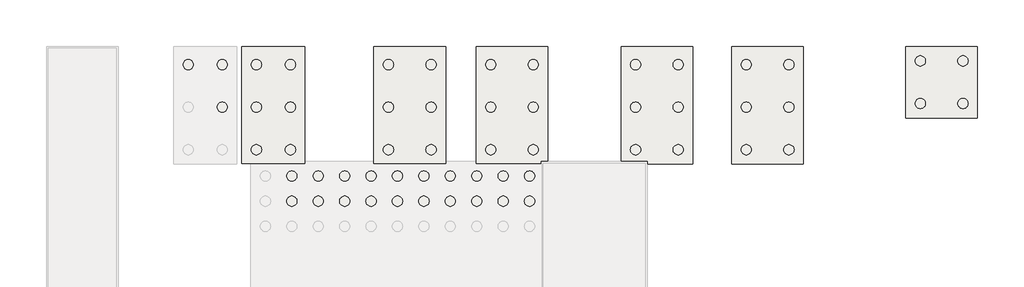
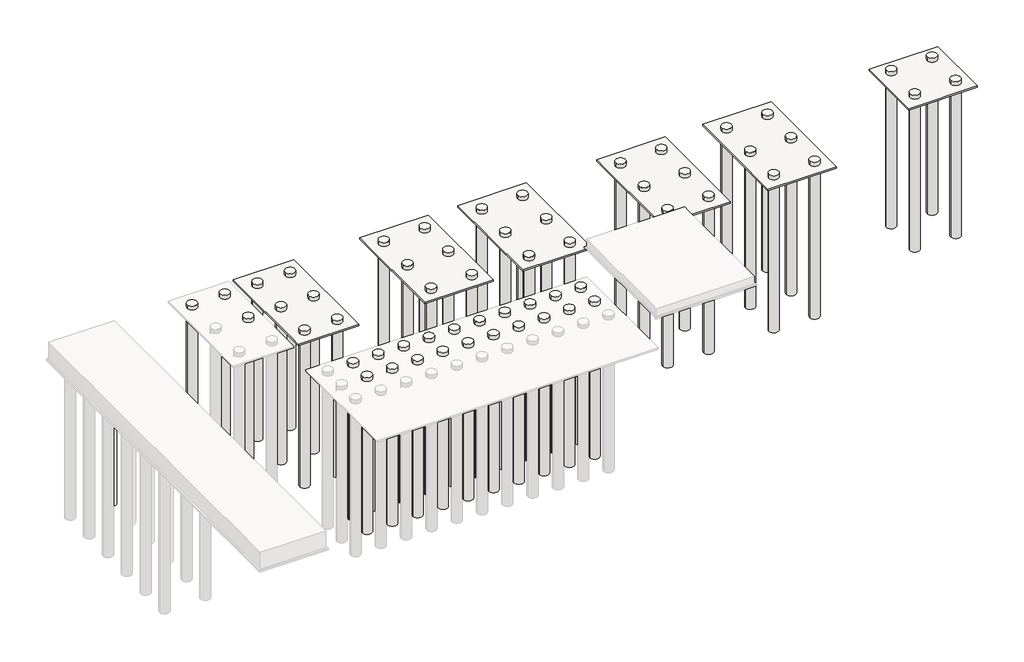
# One storey, part 3 of 3: 64 slabs.
"""IFC4 building model written with IfcOpenShell, lengths in millimetres."""

from ifc_helpers import new_model, si_unit, point, frame, frame_2d, origin, place, context, project, spatial, polyline, circle_curve, trimmed, segment, composite_curve, outline, extrude, faceted_brep, element, save

model = new_model("IFC4")

# Units and contexts
model_context = context("Model", 3, world=origin())
ifc_project = project(units=[si_unit("LENGTHUNIT", "METRE", prefix="MILLI")], contexts=[model_context])

# Site, building, storey
site = spatial("IfcSite", under=ifc_project)
building = spatial("IfcBuilding", under=site)
storey = spatial("IfcBuildingStorey", under=building, Name="B.O.F(FDN)", Elevation=-2500.0279945)

# Slabs
placement = place(None, origin())
element("IfcSlab", 1, ObjectType="H_SF_ACF_Lean_T100", at=placement, inside=storey, context=model_context, shape_type="SweptSolid", body=[
    extrude(outline(polyline([(37900.0, 41319.5208589), (42100.0, 41319.5208589), (42100.0, 34399.5208589), (37900.0, 34399.5208589), (37900.0, 41319.5208589)])), frame((0.0, 0.0, -2600.0279945), z_axis=(0.0, 0.0, 1.0), x_axis=(1.0, 0.0, 0.0)), (0.0, 0.0, 1.0), 100.0),
])
element("IfcSlab", 2, ObjectType="H_SF_ACF_Lean_T100", at=placement, inside=storey, context=model_context, shape_type="SweptSolid", body=[
    extrude(outline(polyline([(48115.0, 41319.5208589), (52315.0, 41319.5208589), (52315.0, 37119.5208589), (48115.0, 37119.5208589), (48115.0, 41319.5208589)])), frame((0.0, 0.0, -2600.0279945), z_axis=(0.0, 0.0, 1.0), x_axis=(1.0, 0.0, 0.0)), (0.0, 0.0, 1.0), 100.0),
])
element("IfcSlab", 3, ObjectType="H_SF_ACF_Lean_T100", at=placement, inside=storey, context=model_context, shape_type="SweptSolid", body=[
    extrude(outline(polyline([(31400.0, 41319.5208589), (35600.0, 41319.5208589), (35600.0, 34399.5208589), (31400.0, 34399.5208589), (31400.0, 41319.5208589)])), frame((0.0, 0.0, -2600.0279945), z_axis=(0.0, 0.0, 1.0), x_axis=(1.0, 0.0, 0.0)), (0.0, 0.0, 1.0), 100.0),
])
element("IfcSlab", 4, ObjectType="H_SF_ACF_Lean_T100", at=placement, inside=storey, context=model_context, shape_type="SweptSolid", body=[
    extrude(outline(polyline([(9150.0, 41319.5208589), (12850.0, 41319.5208589), (12850.0, 34449.5208589), (9150.0, 34449.5208589), (9150.0, 41319.5208589)])), frame((0.0, 0.0, -2600.0279945), z_axis=(0.0, 0.0, 1.0), x_axis=(1.0, 0.0, 0.0)), (0.0, 0.0, 1.0), 100.0),
])
element("IfcSlab", 5, ObjectType="H_SF_ACF_Lean_T100", at=placement, inside=storey, context=model_context, shape_type="SweptSolid", body=[
    extrude(outline(polyline([(21100.0, 41319.5208589), (21100.0, 34449.5208589), (16900.0, 34449.5208589), (16900.0, 41319.5208589), (21100.0, 41319.5208589)])), frame((0.0, 0.0, -2600.0279945), z_axis=(0.0, 0.0, 1.0), x_axis=(1.0, 0.0, 0.0)), (0.0, 0.0, 1.0), 100.0),
])
element("IfcSlab", 6, ObjectType="H_SF_ACF_Lean_T100", at=placement, inside=storey, context=model_context, shape_type="Brep", body=[
    faceted_brep([(27100.0, 41319.5208589, -2600.0279945), (27100.0, 34449.5208589, -2600.0279945), (22900.0, 34449.5208589, -2600.0279945), (22900.0, 41319.5208589, -2600.0279945), (27100.0, 41319.5208589, -2500.0279945), (22900.0, 41319.5208589, -2500.0279945), (22900.0, 34449.5208589, -2500.0279945), (26730.0, 34449.5208589, -2500.0279945), (26780.0, 34449.5208589, -2500.0279945), (27100.0, 34449.5208589, -2500.0279945)], [[[0, 1, 2, 3]], [[4, 5, 6, 7, 8, 9]], [[1, 0, 4, 9]], [[2, 1, 9, 8, 7, 6]], [[3, 2, 6, 5]], [[0, 3, 5, 4]]]),
])
element("IfcSlab", 7, ObjectType="Pile : H_SF_API_Steel Pile D508x12t_L10m", at=placement, inside=storey, context=model_context, shape_type="SweptSolid", body=[
    extrude(outline(composite_curve([segment(trimmed(circle_curve(frame_2d((1035.0, 40249.5208589)), 300.0), [point((1335.0, 40249.5208589))], [point((735.0, 40249.5208589))], False, "CARTESIAN"), True, "CONTINUOUS"), segment(trimmed(circle_curve(frame_2d((1035.0, 40249.5208589)), 300.0), [point((735.0, 40249.5208589))], [point((1335.0, 40249.5208589))], False, "CARTESIAN"), True, "CONTINUOUS")], self_intersect=False)), frame((0.0, 0.0, -13500.0279945), z_axis=(0.0, 0.0, 1.0), x_axis=(1.0, 0.0, 0.0)), (0.0, 0.0, 1.0), 10150.0),
])
element("IfcSlab", 8, ObjectType="Pile : H_SF_API_Steel Pile D508x12t_L10m", at=placement, inside=storey, context=model_context, shape_type="SweptSolid", body=[
    extrude(outline(composite_curve([segment(trimmed(circle_curve(frame_2d((51465.0, 37969.5208589)), 300.0), [point((51765.0, 37969.5208589))], [point((51165.0, 37969.5208589))], False, "CARTESIAN"), True, "CONTINUOUS"), segment(trimmed(circle_curve(frame_2d((51465.0, 37969.5208589)), 300.0), [point((51165.0, 37969.5208589))], [point((51765.0, 37969.5208589))], False, "CARTESIAN"), True, "CONTINUOUS")], self_intersect=False)), frame((0.0, 0.0, -12400.0279945), z_axis=(0.0, 0.0, 1.0), x_axis=(1.0, 0.0, 0.0)), (0.0, 0.0, 1.0), 10150.0),
])
element("IfcSlab", 9, ObjectType="Pile : H_SF_API_Steel Pile D508x12t_L10m", at=placement, inside=storey, context=model_context, shape_type="SweptSolid", body=[
    extrude(outline(composite_curve([segment(trimmed(circle_curve(frame_2d((48965.0, 37969.5208589)), 300.0), [point((48665.0, 37969.5208589))], [point((49265.0, 37969.5208589))], False, "CARTESIAN"), True, "CONTINUOUS"), segment(trimmed(circle_curve(frame_2d((48965.0, 37969.5208589)), 300.0), [point((49265.0, 37969.5208589))], [point((48665.0, 37969.5208589))], False, "CARTESIAN"), True, "CONTINUOUS")], self_intersect=False)), frame((0.0, 0.0, -12400.0279945), z_axis=(0.0, 0.0, 1.0), x_axis=(1.0, 0.0, 0.0)), (0.0, 0.0, 1.0), 10150.0),
])
element("IfcSlab", 10, ObjectType="Pile : H_SF_API_Steel Pile D508x12t_L10m", at=placement, inside=storey, context=model_context, shape_type="SweptSolid", body=[
    extrude(outline(composite_curve([segment(trimmed(circle_curve(frame_2d((51465.0, 40469.5208589)), 300.0), [point((51765.0, 40469.5208589))], [point((51165.0, 40469.5208589))], False, "CARTESIAN"), True, "CONTINUOUS"), segment(trimmed(circle_curve(frame_2d((51465.0, 40469.5208589)), 300.0), [point((51165.0, 40469.5208589))], [point((51765.0, 40469.5208589))], False, "CARTESIAN"), True, "CONTINUOUS")], self_intersect=False)), frame((0.0, 0.0, -12400.0279945), z_axis=(0.0, 0.0, 1.0), x_axis=(1.0, 0.0, 0.0)), (0.0, 0.0, 1.0), 10150.0),
])
element("IfcSlab", 11, ObjectType="Pile : H_SF_API_Steel Pile D508x12t_L10m", at=placement, inside=storey, context=model_context, shape_type="SweptSolid", body=[
    extrude(outline(composite_curve([segment(trimmed(circle_curve(frame_2d((48965.0, 40469.5208589)), 300.0), [point((48665.0, 40469.5208589))], [point((49265.0, 40469.5208589))], False, "CARTESIAN"), True, "CONTINUOUS"), segment(trimmed(circle_curve(frame_2d((48965.0, 40469.5208589)), 300.0), [point((49265.0, 40469.5208589))], [point((48665.0, 40469.5208589))], False, "CARTESIAN"), True, "CONTINUOUS")], self_intersect=False)), frame((0.0, 0.0, -12400.0279945), z_axis=(0.0, 0.0, 1.0), x_axis=(1.0, 0.0, 0.0)), (0.0, 0.0, 1.0), 10150.0),
])
element("IfcSlab", 12, ObjectType="Pile : H_SF_API_Steel Pile D508x12t_L10m", at=placement, inside=storey, context=model_context, shape_type="SweptSolid", body=[
    extrude(outline(composite_curve([segment(trimmed(circle_curve(frame_2d((6000.0, 40249.5208589)), 300.0), [point((5700.0, 40249.5208589))], [point((6300.0, 40249.5208589))], False, "CARTESIAN"), True, "CONTINUOUS"), segment(trimmed(circle_curve(frame_2d((6000.0, 40249.5208589)), 300.0), [point((6300.0, 40249.5208589))], [point((5700.0, 40249.5208589))], False, "CARTESIAN"), True, "CONTINUOUS")], self_intersect=False)), frame((0.0, 0.0, -12400.0279945), z_axis=(0.0, 0.0, 1.0), x_axis=(1.0, 0.0, 0.0)), (0.0, 0.0, 1.0), 10150.0),
])
element("IfcSlab", 13, ObjectType="Pile : H_SF_API_Steel Pile D508x12t_L10m", at=placement, inside=storey, context=model_context, shape_type="SweptSolid", body=[
    extrude(outline(composite_curve([segment(trimmed(circle_curve(frame_2d((8000.0, 40249.5208589)), 300.0), [point((8300.0, 40249.5208589))], [point((7700.0, 40249.5208589))], False, "CARTESIAN"), True, "CONTINUOUS"), segment(trimmed(circle_curve(frame_2d((8000.0, 40249.5208589)), 300.0), [point((7700.0, 40249.5208589))], [point((8300.0, 40249.5208589))], False, "CARTESIAN"), True, "CONTINUOUS")], self_intersect=False)), frame((0.0, 0.0, -12400.0279945), z_axis=(0.0, 0.0, 1.0), x_axis=(1.0, 0.0, 0.0)), (0.0, 0.0, 1.0), 10150.0),
])
element("IfcSlab", 14, ObjectType="Pile : H_SF_API_Steel Pile D508x12t_L10m", at=placement, inside=storey, context=model_context, shape_type="SweptSolid", body=[
    extrude(outline(composite_curve([segment(trimmed(circle_curve(frame_2d((8000.0, 37749.5208589)), 300.0), [point((8300.0, 37749.5208589))], [point((7700.0, 37749.5208589))], False, "CARTESIAN"), True, "CONTINUOUS"), segment(trimmed(circle_curve(frame_2d((8000.0, 37749.5208589)), 300.0), [point((7700.0, 37749.5208589))], [point((8300.0, 37749.5208589))], False, "CARTESIAN"), True, "CONTINUOUS")], self_intersect=False)), frame((0.0, 0.0, -12400.0279945), z_axis=(0.0, 0.0, 1.0), x_axis=(1.0, 0.0, 0.0)), (0.0, 0.0, 1.0), 10150.0),
])
element("IfcSlab", 15, ObjectType="Pile : H_SF_API_Steel Pile D508x12t_L10m", at=placement, inside=storey, context=model_context, shape_type="SweptSolid", body=[
    extrude(outline(composite_curve([segment(trimmed(circle_curve(frame_2d((10000.0, 40249.5208589)), 300.0), [point((9700.0, 40249.5208589))], [point((10300.0, 40249.5208589))], False, "CARTESIAN"), True, "CONTINUOUS"), segment(trimmed(circle_curve(frame_2d((10000.0, 40249.5208589)), 300.0), [point((10300.0, 40249.5208589))], [point((9700.0, 40249.5208589))], False, "CARTESIAN"), True, "CONTINUOUS")], self_intersect=False)), frame((0.0, 0.0, -12400.0279945), z_axis=(0.0, 0.0, 1.0), x_axis=(1.0, 0.0, 0.0)), (0.0, 0.0, 1.0), 10150.0),
])
element("IfcSlab", 16, ObjectType="Pile : H_SF_API_Steel Pile D508x12t_L10m", at=placement, inside=storey, context=model_context, shape_type="SweptSolid", body=[
    extrude(outline(composite_curve([segment(trimmed(circle_curve(frame_2d((12000.0, 40249.5208589)), 300.0), [point((12300.0, 40249.5208589))], [point((11700.0, 40249.5208589))], False, "CARTESIAN"), True, "CONTINUOUS"), segment(trimmed(circle_curve(frame_2d((12000.0, 40249.5208589)), 300.0), [point((11700.0, 40249.5208589))], [point((12300.0, 40249.5208589))], False, "CARTESIAN"), True, "CONTINUOUS")], self_intersect=False)), frame((0.0, 0.0, -12400.0279945), z_axis=(0.0, 0.0, 1.0), x_axis=(1.0, 0.0, 0.0)), (0.0, 0.0, 1.0), 10150.0),
])
element("IfcSlab", 17, ObjectType="Pile : H_SF_API_Steel Pile D508x12t_L10m", at=placement, inside=storey, context=model_context, shape_type="SweptSolid", body=[
    extrude(outline(composite_curve([segment(trimmed(circle_curve(frame_2d((10000.0, 37749.5208589)), 300.0), [point((9700.0, 37749.5208589))], [point((10300.0, 37749.5208589))], False, "CARTESIAN"), True, "CONTINUOUS"), segment(trimmed(circle_curve(frame_2d((10000.0, 37749.5208589)), 300.0), [point((10300.0, 37749.5208589))], [point((9700.0, 37749.5208589))], False, "CARTESIAN"), True, "CONTINUOUS")], self_intersect=False)), frame((0.0, 0.0, -12400.0279945), z_axis=(0.0, 0.0, 1.0), x_axis=(1.0, 0.0, 0.0)), (0.0, 0.0, 1.0), 10150.0),
])
element("IfcSlab", 18, ObjectType="Pile : H_SF_API_Steel Pile D508x12t_L10m", at=placement, inside=storey, context=model_context, shape_type="SweptSolid", body=[
    extrude(outline(composite_curve([segment(trimmed(circle_curve(frame_2d((12000.0, 37749.5208589)), 300.0), [point((12300.0, 37749.5208589))], [point((11700.0, 37749.5208589))], False, "CARTESIAN"), True, "CONTINUOUS"), segment(trimmed(circle_curve(frame_2d((12000.0, 37749.5208589)), 300.0), [point((11700.0, 37749.5208589))], [point((12300.0, 37749.5208589))], False, "CARTESIAN"), True, "CONTINUOUS")], self_intersect=False)), frame((0.0, 0.0, -12400.0279945), z_axis=(0.0, 0.0, 1.0), x_axis=(1.0, 0.0, 0.0)), (0.0, 0.0, 1.0), 10150.0),
])
element("IfcSlab", 19, ObjectType="Pile : H_SF_API_Steel Pile D508x12t_L10m", at=placement, inside=storey, context=model_context, shape_type="SweptSolid", body=[
    extrude(outline(composite_curve([segment(trimmed(circle_curve(frame_2d((10000.0, 35249.5208589)), 300.0), [point((9700.0, 35249.5208589))], [point((10300.0, 35249.5208589))], False, "CARTESIAN"), True, "CONTINUOUS"), segment(trimmed(circle_curve(frame_2d((10000.0, 35249.5208589)), 300.0), [point((10300.0, 35249.5208589))], [point((9700.0, 35249.5208589))], False, "CARTESIAN"), True, "CONTINUOUS")], self_intersect=False)), frame((0.0, 0.0, -12400.0279945), z_axis=(0.0, 0.0, 1.0), x_axis=(1.0, 0.0, 0.0)), (0.0, 0.0, 1.0), 10150.0),
])
element("IfcSlab", 20, ObjectType="Pile : H_SF_API_Steel Pile D508x12t_L10m", at=placement, inside=storey, context=model_context, shape_type="SweptSolid", body=[
    extrude(outline(composite_curve([segment(trimmed(circle_curve(frame_2d((12000.0, 35249.5208589)), 300.0), [point((12300.0, 35249.5208589))], [point((11700.0, 35249.5208589))], False, "CARTESIAN"), True, "CONTINUOUS"), segment(trimmed(circle_curve(frame_2d((12000.0, 35249.5208589)), 300.0), [point((11700.0, 35249.5208589))], [point((12300.0, 35249.5208589))], False, "CARTESIAN"), True, "CONTINUOUS")], self_intersect=False)), frame((0.0, 0.0, -12400.0279945), z_axis=(0.0, 0.0, 1.0), x_axis=(1.0, 0.0, 0.0)), (0.0, 0.0, 1.0), 10150.0),
])
element("IfcSlab", 21, ObjectType="Pile : H_SF_API_Steel Pile D508x12t_L10m", at=placement, inside=storey, context=model_context, shape_type="SweptSolid", body=[
    extrude(outline(composite_curve([segment(trimmed(circle_curve(frame_2d((20250.0, 40249.5208589)), 300.0), [point((20550.0, 40249.5208589))], [point((19950.0, 40249.5208589))], False, "CARTESIAN"), True, "CONTINUOUS"), segment(trimmed(circle_curve(frame_2d((20250.0, 40249.5208589)), 300.0), [point((19950.0, 40249.5208589))], [point((20550.0, 40249.5208589))], False, "CARTESIAN"), True, "CONTINUOUS")], self_intersect=False)), frame((0.0, 0.0, -12400.0279945), z_axis=(0.0, 0.0, 1.0), x_axis=(1.0, 0.0, 0.0)), (0.0, 0.0, 1.0), 10150.0),
])
element("IfcSlab", 22, ObjectType="Pile : H_SF_API_Steel Pile D508x12t_L10m", at=placement, inside=storey, context=model_context, shape_type="SweptSolid", body=[
    extrude(outline(composite_curve([segment(trimmed(circle_curve(frame_2d((17750.0, 40249.5208589)), 300.0), [point((17450.0, 40249.5208589))], [point((18050.0, 40249.5208589))], False, "CARTESIAN"), True, "CONTINUOUS"), segment(trimmed(circle_curve(frame_2d((17750.0, 40249.5208589)), 300.0), [point((18050.0, 40249.5208589))], [point((17450.0, 40249.5208589))], False, "CARTESIAN"), True, "CONTINUOUS")], self_intersect=False)), frame((0.0, 0.0, -12400.0279945), z_axis=(0.0, 0.0, 1.0), x_axis=(1.0, 0.0, 0.0)), (0.0, 0.0, 1.0), 10150.0),
])
element("IfcSlab", 23, ObjectType="Pile : H_SF_API_Steel Pile D508x12t_L10m", at=placement, inside=storey, context=model_context, shape_type="SweptSolid", body=[
    extrude(outline(composite_curve([segment(trimmed(circle_curve(frame_2d((20250.0, 37749.5208589)), 300.0), [point((20550.0, 37749.5208589))], [point((19950.0, 37749.5208589))], False, "CARTESIAN"), True, "CONTINUOUS"), segment(trimmed(circle_curve(frame_2d((20250.0, 37749.5208589)), 300.0), [point((19950.0, 37749.5208589))], [point((20550.0, 37749.5208589))], False, "CARTESIAN"), True, "CONTINUOUS")], self_intersect=False)), frame((0.0, 0.0, -12400.0279945), z_axis=(0.0, 0.0, 1.0), x_axis=(1.0, 0.0, 0.0)), (0.0, 0.0, 1.0), 10150.0),
])
element("IfcSlab", 24, ObjectType="Pile : H_SF_API_Steel Pile D508x12t_L10m", at=placement, inside=storey, context=model_context, shape_type="SweptSolid", body=[
    extrude(outline(composite_curve([segment(trimmed(circle_curve(frame_2d((17750.0, 37749.5208589)), 300.0), [point((17450.0, 37749.5208589))], [point((18050.0, 37749.5208589))], False, "CARTESIAN"), True, "CONTINUOUS"), segment(trimmed(circle_curve(frame_2d((17750.0, 37749.5208589)), 300.0), [point((18050.0, 37749.5208589))], [point((17450.0, 37749.5208589))], False, "CARTESIAN"), True, "CONTINUOUS")], self_intersect=False)), frame((0.0, 0.0, -12400.0279945), z_axis=(0.0, 0.0, 1.0), x_axis=(1.0, 0.0, 0.0)), (0.0, 0.0, 1.0), 10150.0),
])
element("IfcSlab", 25, ObjectType="Pile : H_SF_API_Steel Pile D508x12t_L10m", at=placement, inside=storey, context=model_context, shape_type="SweptSolid", body=[
    extrude(outline(composite_curve([segment(trimmed(circle_curve(frame_2d((20250.0, 35249.5208589)), 300.0), [point((20550.0, 35249.5208589))], [point((19950.0, 35249.5208589))], False, "CARTESIAN"), True, "CONTINUOUS"), segment(trimmed(circle_curve(frame_2d((20250.0, 35249.5208589)), 300.0), [point((19950.0, 35249.5208589))], [point((20550.0, 35249.5208589))], False, "CARTESIAN"), True, "CONTINUOUS")], self_intersect=False)), frame((0.0, 0.0, -12400.0279945), z_axis=(0.0, 0.0, 1.0), x_axis=(1.0, 0.0, 0.0)), (0.0, 0.0, 1.0), 10150.0),
])
element("IfcSlab", 26, ObjectType="Pile : H_SF_API_Steel Pile D508x12t_L10m", at=placement, inside=storey, context=model_context, shape_type="SweptSolid", body=[
    extrude(outline(composite_curve([segment(trimmed(circle_curve(frame_2d((17750.0, 35249.5208589)), 300.0), [point((17450.0, 35249.5208589))], [point((18050.0, 35249.5208589))], False, "CARTESIAN"), True, "CONTINUOUS"), segment(trimmed(circle_curve(frame_2d((17750.0, 35249.5208589)), 300.0), [point((18050.0, 35249.5208589))], [point((17450.0, 35249.5208589))], False, "CARTESIAN"), True, "CONTINUOUS")], self_intersect=False)), frame((0.0, 0.0, -12400.0279945), z_axis=(0.0, 0.0, 1.0), x_axis=(1.0, 0.0, 0.0)), (0.0, 0.0, 1.0), 10150.0),
])
element("IfcSlab", 27, ObjectType="Pile : H_SF_API_Steel Pile D508x12t_L10m", at=placement, inside=storey, context=model_context, shape_type="SweptSolid", body=[
    extrude(outline(composite_curve([segment(trimmed(circle_curve(frame_2d((26250.0, 40249.5208589)), 300.0), [point((26550.0, 40249.5208589))], [point((25950.0, 40249.5208589))], False, "CARTESIAN"), True, "CONTINUOUS"), segment(trimmed(circle_curve(frame_2d((26250.0, 40249.5208589)), 300.0), [point((25950.0, 40249.5208589))], [point((26550.0, 40249.5208589))], False, "CARTESIAN"), True, "CONTINUOUS")], self_intersect=False)), frame((0.0, 0.0, -12400.0279945), z_axis=(0.0, 0.0, 1.0), x_axis=(1.0, 0.0, 0.0)), (0.0, 0.0, 1.0), 10150.0),
])
element("IfcSlab", 28, ObjectType="Pile : H_SF_API_Steel Pile D508x12t_L10m", at=placement, inside=storey, context=model_context, shape_type="SweptSolid", body=[
    extrude(outline(composite_curve([segment(trimmed(circle_curve(frame_2d((23750.0, 40249.5208589)), 300.0), [point((23450.0, 40249.5208589))], [point((24050.0, 40249.5208589))], False, "CARTESIAN"), True, "CONTINUOUS"), segment(trimmed(circle_curve(frame_2d((23750.0, 40249.5208589)), 300.0), [point((24050.0, 40249.5208589))], [point((23450.0, 40249.5208589))], False, "CARTESIAN"), True, "CONTINUOUS")], self_intersect=False)), frame((0.0, 0.0, -12400.0279945), z_axis=(0.0, 0.0, 1.0), x_axis=(1.0, 0.0, 0.0)), (0.0, 0.0, 1.0), 10150.0),
])
element("IfcSlab", 29, ObjectType="Pile : H_SF_API_Steel Pile D508x12t_L10m", at=placement, inside=storey, context=model_context, shape_type="SweptSolid", body=[
    extrude(outline(composite_curve([segment(trimmed(circle_curve(frame_2d((26250.0, 37749.5208589)), 300.0), [point((26550.0, 37749.5208589))], [point((25950.0, 37749.5208589))], False, "CARTESIAN"), True, "CONTINUOUS"), segment(trimmed(circle_curve(frame_2d((26250.0, 37749.5208589)), 300.0), [point((25950.0, 37749.5208589))], [point((26550.0, 37749.5208589))], False, "CARTESIAN"), True, "CONTINUOUS")], self_intersect=False)), frame((0.0, 0.0, -12400.0279945), z_axis=(0.0, 0.0, 1.0), x_axis=(1.0, 0.0, 0.0)), (0.0, 0.0, 1.0), 10150.0),
])
element("IfcSlab", 30, ObjectType="Pile : H_SF_API_Steel Pile D508x12t_L10m", at=placement, inside=storey, context=model_context, shape_type="SweptSolid", body=[
    extrude(outline(composite_curve([segment(trimmed(circle_curve(frame_2d((23750.0, 37749.5208589)), 300.0), [point((23450.0, 37749.5208589))], [point((24050.0, 37749.5208589))], False, "CARTESIAN"), True, "CONTINUOUS"), segment(trimmed(circle_curve(frame_2d((23750.0, 37749.5208589)), 300.0), [point((24050.0, 37749.5208589))], [point((23450.0, 37749.5208589))], False, "CARTESIAN"), True, "CONTINUOUS")], self_intersect=False)), frame((0.0, 0.0, -12400.0279945), z_axis=(0.0, 0.0, 1.0), x_axis=(1.0, 0.0, 0.0)), (0.0, 0.0, 1.0), 10150.0),
])
element("IfcSlab", 31, ObjectType="Pile : H_SF_API_Steel Pile D508x12t_L10m", at=placement, inside=storey, context=model_context, shape_type="SweptSolid", body=[
    extrude(outline(composite_curve([segment(trimmed(circle_curve(frame_2d((26250.0, 35249.5208589)), 300.0), [point((26550.0, 35249.5208589))], [point((25950.0, 35249.5208589))], False, "CARTESIAN"), True, "CONTINUOUS"), segment(trimmed(circle_curve(frame_2d((26250.0, 35249.5208589)), 300.0), [point((25950.0, 35249.5208589))], [point((26550.0, 35249.5208589))], False, "CARTESIAN"), True, "CONTINUOUS")], self_intersect=False)), frame((0.0, 0.0, -12400.0279945), z_axis=(0.0, 0.0, 1.0), x_axis=(1.0, 0.0, 0.0)), (0.0, 0.0, 1.0), 10150.0),
])
element("IfcSlab", 32, ObjectType="Pile : H_SF_API_Steel Pile D508x12t_L10m", at=placement, inside=storey, context=model_context, shape_type="SweptSolid", body=[
    extrude(outline(composite_curve([segment(trimmed(circle_curve(frame_2d((23750.0, 35249.5208589)), 300.0), [point((23450.0, 35249.5208589))], [point((24050.0, 35249.5208589))], False, "CARTESIAN"), True, "CONTINUOUS"), segment(trimmed(circle_curve(frame_2d((23750.0, 35249.5208589)), 300.0), [point((24050.0, 35249.5208589))], [point((23450.0, 35249.5208589))], False, "CARTESIAN"), True, "CONTINUOUS")], self_intersect=False)), frame((0.0, 0.0, -12400.0279945), z_axis=(0.0, 0.0, 1.0), x_axis=(1.0, 0.0, 0.0)), (0.0, 0.0, 1.0), 10150.0),
])
element("IfcSlab", 33, ObjectType="Pile : H_SF_API_Steel Pile D508x12t_L10m", at=placement, inside=storey, context=model_context, shape_type="SweptSolid", body=[
    extrude(outline(composite_curve([segment(trimmed(circle_curve(frame_2d((34750.0, 40249.5208589)), 300.0), [point((35050.0, 40249.5208589))], [point((34450.0, 40249.5208589))], False, "CARTESIAN"), True, "CONTINUOUS"), segment(trimmed(circle_curve(frame_2d((34750.0, 40249.5208589)), 300.0), [point((34450.0, 40249.5208589))], [point((35050.0, 40249.5208589))], False, "CARTESIAN"), True, "CONTINUOUS")], self_intersect=False)), frame((0.0, 0.0, -12400.0279945), z_axis=(0.0, 0.0, 1.0), x_axis=(1.0, 0.0, 0.0)), (0.0, 0.0, 1.0), 10150.0),
])
element("IfcSlab", 34, ObjectType="Pile : H_SF_API_Steel Pile D508x12t_L10m", at=placement, inside=storey, context=model_context, shape_type="SweptSolid", body=[
    extrude(outline(composite_curve([segment(trimmed(circle_curve(frame_2d((32250.0, 40249.5208589)), 300.0), [point((31950.0, 40249.5208589))], [point((32550.0, 40249.5208589))], False, "CARTESIAN"), True, "CONTINUOUS"), segment(trimmed(circle_curve(frame_2d((32250.0, 40249.5208589)), 300.0), [point((32550.0, 40249.5208589))], [point((31950.0, 40249.5208589))], False, "CARTESIAN"), True, "CONTINUOUS")], self_intersect=False)), frame((0.0, 0.0, -12400.0279945), z_axis=(0.0, 0.0, 1.0), x_axis=(1.0, 0.0, 0.0)), (0.0, 0.0, 1.0), 10150.0),
])
element("IfcSlab", 35, ObjectType="Pile : H_SF_API_Steel Pile D508x12t_L10m", at=placement, inside=storey, context=model_context, shape_type="SweptSolid", body=[
    extrude(outline(composite_curve([segment(trimmed(circle_curve(frame_2d((34750.0, 37749.5208589)), 300.0), [point((35050.0, 37749.5208589))], [point((34450.0, 37749.5208589))], False, "CARTESIAN"), True, "CONTINUOUS"), segment(trimmed(circle_curve(frame_2d((34750.0, 37749.5208589)), 300.0), [point((34450.0, 37749.5208589))], [point((35050.0, 37749.5208589))], False, "CARTESIAN"), True, "CONTINUOUS")], self_intersect=False)), frame((0.0, 0.0, -12400.0279945), z_axis=(0.0, 0.0, 1.0), x_axis=(1.0, 0.0, 0.0)), (0.0, 0.0, 1.0), 10150.0),
])
element("IfcSlab", 36, ObjectType="Pile : H_SF_API_Steel Pile D508x12t_L10m", at=placement, inside=storey, context=model_context, shape_type="SweptSolid", body=[
    extrude(outline(composite_curve([segment(trimmed(circle_curve(frame_2d((32250.0, 37749.5208589)), 300.0), [point((31950.0, 37749.5208589))], [point((32550.0, 37749.5208589))], False, "CARTESIAN"), True, "CONTINUOUS"), segment(trimmed(circle_curve(frame_2d((32250.0, 37749.5208589)), 300.0), [point((32550.0, 37749.5208589))], [point((31950.0, 37749.5208589))], False, "CARTESIAN"), True, "CONTINUOUS")], self_intersect=False)), frame((0.0, 0.0, -12400.0279945), z_axis=(0.0, 0.0, 1.0), x_axis=(1.0, 0.0, 0.0)), (0.0, 0.0, 1.0), 10150.0),
])
element("IfcSlab", 37, ObjectType="Pile : H_SF_API_Steel Pile D508x12t_L10m", at=placement, inside=storey, context=model_context, shape_type="SweptSolid", body=[
    extrude(outline(composite_curve([segment(trimmed(circle_curve(frame_2d((34750.0, 35249.5208589)), 300.0), [point((35050.0, 35249.5208589))], [point((34450.0, 35249.5208589))], False, "CARTESIAN"), True, "CONTINUOUS"), segment(trimmed(circle_curve(frame_2d((34750.0, 35249.5208589)), 300.0), [point((34450.0, 35249.5208589))], [point((35050.0, 35249.5208589))], False, "CARTESIAN"), True, "CONTINUOUS")], self_intersect=False)), frame((0.0, 0.0, -12400.0279945), z_axis=(0.0, 0.0, 1.0), x_axis=(1.0, 0.0, 0.0)), (0.0, 0.0, 1.0), 10150.0),
])
element("IfcSlab", 38, ObjectType="Pile : H_SF_API_Steel Pile D508x12t_L10m", at=placement, inside=storey, context=model_context, shape_type="SweptSolid", body=[
    extrude(outline(composite_curve([segment(trimmed(circle_curve(frame_2d((32250.0, 35249.5208589)), 300.0), [point((31950.0, 35249.5208589))], [point((32550.0, 35249.5208589))], False, "CARTESIAN"), True, "CONTINUOUS"), segment(trimmed(circle_curve(frame_2d((32250.0, 35249.5208589)), 300.0), [point((32550.0, 35249.5208589))], [point((31950.0, 35249.5208589))], False, "CARTESIAN"), True, "CONTINUOUS")], self_intersect=False)), frame((0.0, 0.0, -12400.0279945), z_axis=(0.0, 0.0, 1.0), x_axis=(1.0, 0.0, 0.0)), (0.0, 0.0, 1.0), 10150.0),
])
element("IfcSlab", 39, ObjectType="Pile : H_SF_API_Steel Pile D508x12t_L10m", at=placement, inside=storey, context=model_context, shape_type="SweptSolid", body=[
    extrude(outline(composite_curve([segment(trimmed(circle_curve(frame_2d((41250.0, 40249.5208589)), 300.0), [point((41550.0, 40249.5208589))], [point((40950.0, 40249.5208589))], False, "CARTESIAN"), True, "CONTINUOUS"), segment(trimmed(circle_curve(frame_2d((41250.0, 40249.5208589)), 300.0), [point((40950.0, 40249.5208589))], [point((41550.0, 40249.5208589))], False, "CARTESIAN"), True, "CONTINUOUS")], self_intersect=False)), frame((0.0, 0.0, -12400.0279945), z_axis=(0.0, 0.0, 1.0), x_axis=(1.0, 0.0, 0.0)), (0.0, 0.0, 1.0), 10150.0),
])
element("IfcSlab", 40, ObjectType="Pile : H_SF_API_Steel Pile D508x12t_L10m", at=placement, inside=storey, context=model_context, shape_type="SweptSolid", body=[
    extrude(outline(composite_curve([segment(trimmed(circle_curve(frame_2d((38750.0, 40249.5208589)), 300.0), [point((38450.0, 40249.5208589))], [point((39050.0, 40249.5208589))], False, "CARTESIAN"), True, "CONTINUOUS"), segment(trimmed(circle_curve(frame_2d((38750.0, 40249.5208589)), 300.0), [point((39050.0, 40249.5208589))], [point((38450.0, 40249.5208589))], False, "CARTESIAN"), True, "CONTINUOUS")], self_intersect=False)), frame((0.0, 0.0, -12400.0279945), z_axis=(0.0, 0.0, 1.0), x_axis=(1.0, 0.0, 0.0)), (0.0, 0.0, 1.0), 10150.0),
])
element("IfcSlab", 41, ObjectType="Pile : H_SF_API_Steel Pile D508x12t_L10m", at=placement, inside=storey, context=model_context, shape_type="SweptSolid", body=[
    extrude(outline(composite_curve([segment(trimmed(circle_curve(frame_2d((41250.0, 37749.5208589)), 300.0), [point((41550.0, 37749.5208589))], [point((40950.0, 37749.5208589))], False, "CARTESIAN"), True, "CONTINUOUS"), segment(trimmed(circle_curve(frame_2d((41250.0, 37749.5208589)), 300.0), [point((40950.0, 37749.5208589))], [point((41550.0, 37749.5208589))], False, "CARTESIAN"), True, "CONTINUOUS")], self_intersect=False)), frame((0.0, 0.0, -12400.0279945), z_axis=(0.0, 0.0, 1.0), x_axis=(1.0, 0.0, 0.0)), (0.0, 0.0, 1.0), 10150.0),
])
element("IfcSlab", 42, ObjectType="Pile : H_SF_API_Steel Pile D508x12t_L10m", at=placement, inside=storey, context=model_context, shape_type="SweptSolid", body=[
    extrude(outline(composite_curve([segment(trimmed(circle_curve(frame_2d((38750.0, 37749.5208589)), 300.0), [point((38450.0, 37749.5208589))], [point((39050.0, 37749.5208589))], False, "CARTESIAN"), True, "CONTINUOUS"), segment(trimmed(circle_curve(frame_2d((38750.0, 37749.5208589)), 300.0), [point((39050.0, 37749.5208589))], [point((38450.0, 37749.5208589))], False, "CARTESIAN"), True, "CONTINUOUS")], self_intersect=False)), frame((0.0, 0.0, -12400.0279945), z_axis=(0.0, 0.0, 1.0), x_axis=(1.0, 0.0, 0.0)), (0.0, 0.0, 1.0), 10150.0),
])
element("IfcSlab", 43, ObjectType="Pile : H_SF_API_Steel Pile D508x12t_L10m", at=placement, inside=storey, context=model_context, shape_type="SweptSolid", body=[
    extrude(outline(composite_curve([segment(trimmed(circle_curve(frame_2d((41250.0, 35249.5208589)), 300.0), [point((41550.0, 35249.5208589))], [point((40950.0, 35249.5208589))], False, "CARTESIAN"), True, "CONTINUOUS"), segment(trimmed(circle_curve(frame_2d((41250.0, 35249.5208589)), 300.0), [point((40950.0, 35249.5208589))], [point((41550.0, 35249.5208589))], False, "CARTESIAN"), True, "CONTINUOUS")], self_intersect=False)), frame((0.0, 0.0, -12400.0279945), z_axis=(0.0, 0.0, 1.0), x_axis=(1.0, 0.0, 0.0)), (0.0, 0.0, 1.0), 10150.0),
])
element("IfcSlab", 44, ObjectType="Pile : H_SF_API_Steel Pile D508x12t_L10m", at=placement, inside=storey, context=model_context, shape_type="SweptSolid", body=[
    extrude(outline(composite_curve([segment(trimmed(circle_curve(frame_2d((38750.0, 35249.5208589)), 300.0), [point((38450.0, 35249.5208589))], [point((39050.0, 35249.5208589))], False, "CARTESIAN"), True, "CONTINUOUS"), segment(trimmed(circle_curve(frame_2d((38750.0, 35249.5208589)), 300.0), [point((39050.0, 35249.5208589))], [point((38450.0, 35249.5208589))], False, "CARTESIAN"), True, "CONTINUOUS")], self_intersect=False)), frame((0.0, 0.0, -12400.0279945), z_axis=(0.0, 0.0, 1.0), x_axis=(1.0, 0.0, 0.0)), (0.0, 0.0, 1.0), 10150.0),
])
element("IfcSlab", 45, ObjectType="Pile : H_SF_API_Steel Pile D508x12t_L10m", at=placement, inside=storey, context=model_context, shape_type="SweptSolid", body=[
    extrude(outline(composite_curve([segment(trimmed(circle_curve(frame_2d((26030.0, 33699.5208589)), 300.0), [point((26330.0, 33699.5208589))], [point((25730.0, 33699.5208589))], False, "CARTESIAN"), True, "CONTINUOUS"), segment(trimmed(circle_curve(frame_2d((26030.0, 33699.5208589)), 300.0), [point((25730.0, 33699.5208589))], [point((26330.0, 33699.5208589))], False, "CARTESIAN"), True, "CONTINUOUS")], self_intersect=False)), frame((0.0, 0.0, -14300.0279945), z_axis=(0.0, 0.0, 1.0), x_axis=(1.0, 0.0, 0.0)), (0.0, 0.0, 1.0), 10150.0),
])
element("IfcSlab", 46, ObjectType="Pile : H_SF_API_Steel Pile D508x12t_L10m", at=placement, inside=storey, context=model_context, shape_type="SweptSolid", body=[
    extrude(outline(composite_curve([segment(trimmed(circle_curve(frame_2d((26030.0, 32224.5208589)), 300.0), [point((26330.0, 32224.5208589))], [point((25730.0, 32224.5208589))], False, "CARTESIAN"), True, "CONTINUOUS"), segment(trimmed(circle_curve(frame_2d((26030.0, 32224.5208589)), 300.0), [point((25730.0, 32224.5208589))], [point((26330.0, 32224.5208589))], False, "CARTESIAN"), True, "CONTINUOUS")], self_intersect=False)), frame((0.0, 0.0, -14300.0279945), z_axis=(0.0, 0.0, 1.0), x_axis=(1.0, 0.0, 0.0)), (0.0, 0.0, 1.0), 10150.0),
])
element("IfcSlab", 47, ObjectType="Pile : H_SF_API_Steel Pile D508x12t_L10m", at=placement, inside=storey, context=model_context, shape_type="SweptSolid", body=[
    extrude(outline(composite_curve([segment(trimmed(circle_curve(frame_2d((24480.0, 33699.5208589)), 300.0), [point((24780.0, 33699.5208589))], [point((24180.0, 33699.5208589))], False, "CARTESIAN"), True, "CONTINUOUS"), segment(trimmed(circle_curve(frame_2d((24480.0, 33699.5208589)), 300.0), [point((24180.0, 33699.5208589))], [point((24780.0, 33699.5208589))], False, "CARTESIAN"), True, "CONTINUOUS")], self_intersect=False)), frame((0.0, 0.0, -14300.0279945), z_axis=(0.0, 0.0, 1.0), x_axis=(1.0, 0.0, 0.0)), (0.0, 0.0, 1.0), 10150.0),
])
element("IfcSlab", 48, ObjectType="Pile : H_SF_API_Steel Pile D508x12t_L10m", at=placement, inside=storey, context=model_context, shape_type="SweptSolid", body=[
    extrude(outline(composite_curve([segment(trimmed(circle_curve(frame_2d((24480.0, 32224.5208589)), 300.0), [point((24780.0, 32224.5208589))], [point((24180.0, 32224.5208589))], False, "CARTESIAN"), True, "CONTINUOUS"), segment(trimmed(circle_curve(frame_2d((24480.0, 32224.5208589)), 300.0), [point((24180.0, 32224.5208589))], [point((24780.0, 32224.5208589))], False, "CARTESIAN"), True, "CONTINUOUS")], self_intersect=False)), frame((0.0, 0.0, -14300.0279945), z_axis=(0.0, 0.0, 1.0), x_axis=(1.0, 0.0, 0.0)), (0.0, 0.0, 1.0), 10150.0),
])
element("IfcSlab", 49, ObjectType="Pile : H_SF_API_Steel Pile D508x12t_L10m", at=placement, inside=storey, context=model_context, shape_type="SweptSolid", body=[
    extrude(outline(composite_curve([segment(trimmed(circle_curve(frame_2d((22930.0, 33699.5208589)), 300.0), [point((23230.0, 33699.5208589))], [point((22630.0, 33699.5208589))], False, "CARTESIAN"), True, "CONTINUOUS"), segment(trimmed(circle_curve(frame_2d((22930.0, 33699.5208589)), 300.0), [point((22630.0, 33699.5208589))], [point((23230.0, 33699.5208589))], False, "CARTESIAN"), True, "CONTINUOUS")], self_intersect=False)), frame((0.0, 0.0, -14300.0279945), z_axis=(0.0, 0.0, 1.0), x_axis=(1.0, 0.0, 0.0)), (0.0, 0.0, 1.0), 10150.0),
])
element("IfcSlab", 50, ObjectType="Pile : H_SF_API_Steel Pile D508x12t_L10m", at=placement, inside=storey, context=model_context, shape_type="SweptSolid", body=[
    extrude(outline(composite_curve([segment(trimmed(circle_curve(frame_2d((22930.0, 32224.5208589)), 300.0), [point((23230.0, 32224.5208589))], [point((22630.0, 32224.5208589))], False, "CARTESIAN"), True, "CONTINUOUS"), segment(trimmed(circle_curve(frame_2d((22930.0, 32224.5208589)), 300.0), [point((22630.0, 32224.5208589))], [point((23230.0, 32224.5208589))], False, "CARTESIAN"), True, "CONTINUOUS")], self_intersect=False)), frame((0.0, 0.0, -14300.0279945), z_axis=(0.0, 0.0, 1.0), x_axis=(1.0, 0.0, 0.0)), (0.0, 0.0, 1.0), 10150.0),
])
element("IfcSlab", 51, ObjectType="Pile : H_SF_API_Steel Pile D508x12t_L10m", at=placement, inside=storey, context=model_context, shape_type="SweptSolid", body=[
    extrude(outline(composite_curve([segment(trimmed(circle_curve(frame_2d((21380.0, 33699.5208589)), 300.0), [point((21680.0, 33699.5208589))], [point((21080.0, 33699.5208589))], False, "CARTESIAN"), True, "CONTINUOUS"), segment(trimmed(circle_curve(frame_2d((21380.0, 33699.5208589)), 300.0), [point((21080.0, 33699.5208589))], [point((21680.0, 33699.5208589))], False, "CARTESIAN"), True, "CONTINUOUS")], self_intersect=False)), frame((0.0, 0.0, -14300.0279945), z_axis=(0.0, 0.0, 1.0), x_axis=(1.0, 0.0, 0.0)), (0.0, 0.0, 1.0), 10150.0),
])
element("IfcSlab", 52, ObjectType="Pile : H_SF_API_Steel Pile D508x12t_L10m", at=placement, inside=storey, context=model_context, shape_type="SweptSolid", body=[
    extrude(outline(composite_curve([segment(trimmed(circle_curve(frame_2d((21380.0, 32224.5208589)), 300.0), [point((21680.0, 32224.5208589))], [point((21080.0, 32224.5208589))], False, "CARTESIAN"), True, "CONTINUOUS"), segment(trimmed(circle_curve(frame_2d((21380.0, 32224.5208589)), 300.0), [point((21080.0, 32224.5208589))], [point((21680.0, 32224.5208589))], False, "CARTESIAN"), True, "CONTINUOUS")], self_intersect=False)), frame((0.0, 0.0, -14300.0279945), z_axis=(0.0, 0.0, 1.0), x_axis=(1.0, 0.0, 0.0)), (0.0, 0.0, 1.0), 10150.0),
])
element("IfcSlab", 53, ObjectType="Pile : H_SF_API_Steel Pile D508x12t_L10m", at=placement, inside=storey, context=model_context, shape_type="SweptSolid", body=[
    extrude(outline(composite_curve([segment(trimmed(circle_curve(frame_2d((19830.0, 33699.5208589)), 300.0), [point((20130.0, 33699.5208589))], [point((19530.0, 33699.5208589))], False, "CARTESIAN"), True, "CONTINUOUS"), segment(trimmed(circle_curve(frame_2d((19830.0, 33699.5208589)), 300.0), [point((19530.0, 33699.5208589))], [point((20130.0, 33699.5208589))], False, "CARTESIAN"), True, "CONTINUOUS")], self_intersect=False)), frame((0.0, 0.0, -14300.0279945), z_axis=(0.0, 0.0, 1.0), x_axis=(1.0, 0.0, 0.0)), (0.0, 0.0, 1.0), 10150.0),
])
element("IfcSlab", 54, ObjectType="Pile : H_SF_API_Steel Pile D508x12t_L10m", at=placement, inside=storey, context=model_context, shape_type="SweptSolid", body=[
    extrude(outline(composite_curve([segment(trimmed(circle_curve(frame_2d((19830.0, 32224.5208589)), 300.0), [point((20130.0, 32224.5208589))], [point((19530.0, 32224.5208589))], False, "CARTESIAN"), True, "CONTINUOUS"), segment(trimmed(circle_curve(frame_2d((19830.0, 32224.5208589)), 300.0), [point((19530.0, 32224.5208589))], [point((20130.0, 32224.5208589))], False, "CARTESIAN"), True, "CONTINUOUS")], self_intersect=False)), frame((0.0, 0.0, -14300.0279945), z_axis=(0.0, 0.0, 1.0), x_axis=(1.0, 0.0, 0.0)), (0.0, 0.0, 1.0), 10150.0),
])
element("IfcSlab", 55, ObjectType="Pile : H_SF_API_Steel Pile D508x12t_L10m", at=placement, inside=storey, context=model_context, shape_type="SweptSolid", body=[
    extrude(outline(composite_curve([segment(trimmed(circle_curve(frame_2d((18280.0, 33699.5208589)), 300.0), [point((18580.0, 33699.5208589))], [point((17980.0, 33699.5208589))], False, "CARTESIAN"), True, "CONTINUOUS"), segment(trimmed(circle_curve(frame_2d((18280.0, 33699.5208589)), 300.0), [point((17980.0, 33699.5208589))], [point((18580.0, 33699.5208589))], False, "CARTESIAN"), True, "CONTINUOUS")], self_intersect=False)), frame((0.0, 0.0, -14300.0279945), z_axis=(0.0, 0.0, 1.0), x_axis=(1.0, 0.0, 0.0)), (0.0, 0.0, 1.0), 10150.0),
])
element("IfcSlab", 56, ObjectType="Pile : H_SF_API_Steel Pile D508x12t_L10m", at=placement, inside=storey, context=model_context, shape_type="SweptSolid", body=[
    extrude(outline(composite_curve([segment(trimmed(circle_curve(frame_2d((18280.0, 32224.5208589)), 300.0), [point((18580.0, 32224.5208589))], [point((17980.0, 32224.5208589))], False, "CARTESIAN"), True, "CONTINUOUS"), segment(trimmed(circle_curve(frame_2d((18280.0, 32224.5208589)), 300.0), [point((17980.0, 32224.5208589))], [point((18580.0, 32224.5208589))], False, "CARTESIAN"), True, "CONTINUOUS")], self_intersect=False)), frame((0.0, 0.0, -14300.0279945), z_axis=(0.0, 0.0, 1.0), x_axis=(1.0, 0.0, 0.0)), (0.0, 0.0, 1.0), 10150.0),
])
element("IfcSlab", 57, ObjectType="Pile : H_SF_API_Steel Pile D508x12t_L10m", at=placement, inside=storey, context=model_context, shape_type="SweptSolid", body=[
    extrude(outline(composite_curve([segment(trimmed(circle_curve(frame_2d((16730.0, 33699.5208589)), 300.0), [point((17030.0, 33699.5208589))], [point((16430.0, 33699.5208589))], False, "CARTESIAN"), True, "CONTINUOUS"), segment(trimmed(circle_curve(frame_2d((16730.0, 33699.5208589)), 300.0), [point((16430.0, 33699.5208589))], [point((17030.0, 33699.5208589))], False, "CARTESIAN"), True, "CONTINUOUS")], self_intersect=False)), frame((0.0, 0.0, -14300.0279945), z_axis=(0.0, 0.0, 1.0), x_axis=(1.0, 0.0, 0.0)), (0.0, 0.0, 1.0), 10150.0),
])
element("IfcSlab", 58, ObjectType="Pile : H_SF_API_Steel Pile D508x12t_L10m", at=placement, inside=storey, context=model_context, shape_type="SweptSolid", body=[
    extrude(outline(composite_curve([segment(trimmed(circle_curve(frame_2d((16730.0, 32224.5208589)), 300.0), [point((17030.0, 32224.5208589))], [point((16430.0, 32224.5208589))], False, "CARTESIAN"), True, "CONTINUOUS"), segment(trimmed(circle_curve(frame_2d((16730.0, 32224.5208589)), 300.0), [point((16430.0, 32224.5208589))], [point((17030.0, 32224.5208589))], False, "CARTESIAN"), True, "CONTINUOUS")], self_intersect=False)), frame((0.0, 0.0, -14300.0279945), z_axis=(0.0, 0.0, 1.0), x_axis=(1.0, 0.0, 0.0)), (0.0, 0.0, 1.0), 10150.0),
])
element("IfcSlab", 59, ObjectType="Pile : H_SF_API_Steel Pile D508x12t_L10m", at=placement, inside=storey, context=model_context, shape_type="SweptSolid", body=[
    extrude(outline(composite_curve([segment(trimmed(circle_curve(frame_2d((15180.0, 33699.5208589)), 300.0), [point((15480.0, 33699.5208589))], [point((14880.0, 33699.5208589))], False, "CARTESIAN"), True, "CONTINUOUS"), segment(trimmed(circle_curve(frame_2d((15180.0, 33699.5208589)), 300.0), [point((14880.0, 33699.5208589))], [point((15480.0, 33699.5208589))], False, "CARTESIAN"), True, "CONTINUOUS")], self_intersect=False)), frame((0.0, 0.0, -14300.0279945), z_axis=(0.0, 0.0, 1.0), x_axis=(1.0, 0.0, 0.0)), (0.0, 0.0, 1.0), 10150.0),
])
element("IfcSlab", 60, ObjectType="Pile : H_SF_API_Steel Pile D508x12t_L10m", at=placement, inside=storey, context=model_context, shape_type="SweptSolid", body=[
    extrude(outline(composite_curve([segment(trimmed(circle_curve(frame_2d((15180.0, 32224.5208589)), 300.0), [point((15480.0, 32224.5208589))], [point((14880.0, 32224.5208589))], False, "CARTESIAN"), True, "CONTINUOUS"), segment(trimmed(circle_curve(frame_2d((15180.0, 32224.5208589)), 300.0), [point((14880.0, 32224.5208589))], [point((15480.0, 32224.5208589))], False, "CARTESIAN"), True, "CONTINUOUS")], self_intersect=False)), frame((0.0, 0.0, -14300.0279945), z_axis=(0.0, 0.0, 1.0), x_axis=(1.0, 0.0, 0.0)), (0.0, 0.0, 1.0), 10150.0),
])
element("IfcSlab", 61, ObjectType="Pile : H_SF_API_Steel Pile D508x12t_L10m", at=placement, inside=storey, context=model_context, shape_type="SweptSolid", body=[
    extrude(outline(composite_curve([segment(trimmed(circle_curve(frame_2d((13630.0, 33699.5208589)), 300.0), [point((13930.0, 33699.5208589))], [point((13330.0, 33699.5208589))], False, "CARTESIAN"), True, "CONTINUOUS"), segment(trimmed(circle_curve(frame_2d((13630.0, 33699.5208589)), 300.0), [point((13330.0, 33699.5208589))], [point((13930.0, 33699.5208589))], False, "CARTESIAN"), True, "CONTINUOUS")], self_intersect=False)), frame((0.0, 0.0, -14300.0279945), z_axis=(0.0, 0.0, 1.0), x_axis=(1.0, 0.0, 0.0)), (0.0, 0.0, 1.0), 10150.0),
])
element("IfcSlab", 62, ObjectType="Pile : H_SF_API_Steel Pile D508x12t_L10m", at=placement, inside=storey, context=model_context, shape_type="SweptSolid", body=[
    extrude(outline(composite_curve([segment(trimmed(circle_curve(frame_2d((13630.0, 32224.5208589)), 300.0), [point((13930.0, 32224.5208589))], [point((13330.0, 32224.5208589))], False, "CARTESIAN"), True, "CONTINUOUS"), segment(trimmed(circle_curve(frame_2d((13630.0, 32224.5208589)), 300.0), [point((13330.0, 32224.5208589))], [point((13930.0, 32224.5208589))], False, "CARTESIAN"), True, "CONTINUOUS")], self_intersect=False)), frame((0.0, 0.0, -14300.0279945), z_axis=(0.0, 0.0, 1.0), x_axis=(1.0, 0.0, 0.0)), (0.0, 0.0, 1.0), 10150.0),
])
element("IfcSlab", 63, ObjectType="Pile : H_SF_API_Steel Pile D508x12t_L10m", at=placement, inside=storey, context=model_context, shape_type="SweptSolid", body=[
    extrude(outline(composite_curve([segment(trimmed(circle_curve(frame_2d((12080.0, 33699.5208589)), 300.0), [point((12380.0, 33699.5208589))], [point((11780.0, 33699.5208589))], False, "CARTESIAN"), True, "CONTINUOUS"), segment(trimmed(circle_curve(frame_2d((12080.0, 33699.5208589)), 300.0), [point((11780.0, 33699.5208589))], [point((12380.0, 33699.5208589))], False, "CARTESIAN"), True, "CONTINUOUS")], self_intersect=False)), frame((0.0, 0.0, -14300.0279945), z_axis=(0.0, 0.0, 1.0), x_axis=(1.0, 0.0, 0.0)), (0.0, 0.0, 1.0), 10150.0),
])
element("IfcSlab", 64, ObjectType="Pile : H_SF_API_Steel Pile D508x12t_L10m", at=placement, inside=storey, context=model_context, shape_type="SweptSolid", body=[
    extrude(outline(composite_curve([segment(trimmed(circle_curve(frame_2d((12080.0, 32224.5208589)), 300.0), [point((12380.0, 32224.5208589))], [point((11780.0, 32224.5208589))], False, "CARTESIAN"), True, "CONTINUOUS"), segment(trimmed(circle_curve(frame_2d((12080.0, 32224.5208589)), 300.0), [point((11780.0, 32224.5208589))], [point((12380.0, 32224.5208589))], False, "CARTESIAN"), True, "CONTINUOUS")], self_intersect=False)), frame((0.0, 0.0, -14300.0279945), z_axis=(0.0, 0.0, 1.0), x_axis=(1.0, 0.0, 0.0)), (0.0, 0.0, 1.0), 10150.0),
])

save(model, "model.ifc")

# Revit data of these elements
# Type "H_SF_ACF_Lean_T100"
#   Type Comments = "구조_콘크리트"
#   H_WM Code_1 = "A03AD034-00004 | Concrete Work | Substructure Work | Lean Concrete (including Form work) | Cement Type-1 | 10MPa < F'c (Cylinder Strength) ≤ 20MPa"
#   H_WM Code_2 = "A01ZZ005-00001 | Earth Work | - | Base Course | THK≤150mm | THK=(  )mm | CBR=(  )%"
#   H_WM Code_3 = "A01ZZ006-00001 | Earth Work | - | Subbase Course | Including Compaction of Sub-Grade | THK≤150mm | THK=(  )mm | CBR=(  )% for Subgrade, (  )% for Subbase | Compaction=(  )% for Subgrade, (  )% for Subbase"
#   H_WM Code_4 = "A01ZZ012-00001 | Earth Work | - | PE Sheet (Vapor Barrier) | THK=(  )mm"
#   H_Q'ty Cal Type Tag = "SF-Q3"
#   Layers, outside or top first: 0.1000 m "A03AC034-00004_Lean Concrete (including Form work)" (function 1)
# Type "Pile : H_SF_API_Steel Pile D508x12t_L10m"
#   Type Mark = ""
#   H_WM Code_1 = "A02AA020-00001 | Pile Work | Piling Work | Steel Pipe Pile Work | Direct Driving | Including Pile Connection and Joint Welding Work | D=(  )mm / THK=(  )mm | Pile Length per Hole=(  )M"
#   H_WM Code_2 = "A02AB020-00001 | Pile Work | Pile Head Treatment | Steel Pipe Pile Work | D=(  )mm / THK=(  )mm"
#   H_Q'ty Cal Type Tag = "SF-Q5"
#   Assembly Code = "A1020130"
#   반지름 = 0.3000 m
#   최소 내포 = 0.1500 m
#   Diameter = 0.6000 m
#   Depth = 10.0000 m
#   VISIBLE [instance default] = yes
#   구조 재료 = 콘크리트
# Elements 1, 2, 3, 4 (IfcSlab, "H_SF_ACF_Lean_T100")
#   Comments = ""
#   built-in parameter 1001955 = 3.14159 (stored number, unit not read)
#   Height Offset From Level = 0.0000 m
#   built-in parameter 1001954 = 1
#   Phase Created = New Construction
#   Materials on its faces: "A03AC034-00004_Lean Concrete (including Form work)"
# Elements 5, 6 (IfcSlab, "H_SF_ACF_Lean_T100")
#   Comments = ""
#   Height Offset From Level = 0.0000 m
#   built-in parameter 1001954 = 1
#   Phase Created = New Construction
#   Materials on its faces: "A03AC034-00004_Lean Concrete (including Form work)"
# Element 7 (IfcSlab, "Pile : H_SF_API_Steel Pile D508x12t_L10m")
#   Mark = "102"
#   Phase Created = New Construction
#   Materials on its faces: "금속 - 스틸 - 345MPa"
# Elements 8, 9, 10, 11, 12, 13, 14, 15, 16, 17, 18, 19, 20, 21, 22, 23, 24, 25, 26, 28, 30, 32, 33, 34, 35, 36, 37, 38, 39, 40, 41, 42, 43, 44, 49, 50, 51, 52, 53, 54, 55, 56, 57, 58, 59, 60, 61, 62, 63, 64 (IfcSlab, "Pile : H_SF_API_Steel Pile D508x12t_L10m")
#   Phase Created = New Construction
#   Materials on its faces: "금속 - 스틸 - 345MPa"
# Elements 27, 29, 31, 45, 46, 47, 48 (IfcSlab, "Pile : H_SF_API_Steel Pile D508x12t_L10m")
#   VISIBLE = yes
#   Phase Created = New Construction
#   Materials on its faces: "금속 - 스틸 - 345MPa"
# Materials
#   "A03AC034-00004_Lean Concrete (including Form work)": class "Concrete", colour RGB 176 176 176, transparency 0, Description = "Plain Conc.", Cost = 0
#   "콘크리트": class "*D 철근콘크리트공사", colour RGB 192 192 192, transparency 0, Keynote = "DF", Description = "콘크리트", Cost = 0
#   "금속 - 스틸 - 345MPa": class "금속", colour RGB 247 247 247, transparency 0
